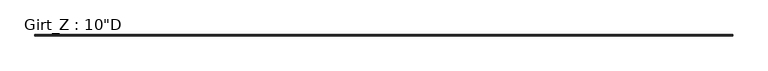
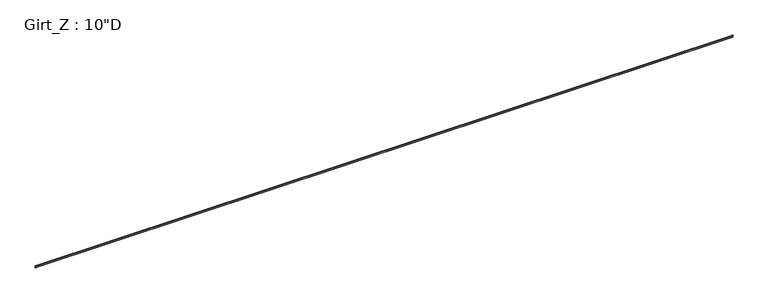
"""IFC4 building model written with IfcOpenShell, lengths in millimetres: beam geometry."""

from ifc_helpers import new_model, si_unit, point, frame, frame_2d, origin, place, context, project, spatial, polyline, circle_curve, trimmed, segment, composite_curve, outline, extrude, source, transform, mapped, element, save


def beam_b1d2936f(model_context):
    return source(origin(), model_context, "Body", "SweptSolid", [
        extrude(outline(composite_curve([segment(polyline([(-77.9859375, 127.0), (-3.3734375, 127.0)]), True, "CONTINUOUS"), segment(trimmed(circle_curve(frame_2d((-3.3734375, 122.2375)), 4.7625), [point((-3.3734375, 127.0))], [point((1.3890625, 122.2375))], False, "CARTESIAN"), True, "CONTINUOUS"), segment(polyline([(1.3890625, 122.2375), (1.3890625, -122.2389339)]), True, "CONTINUOUS"), segment(trimmed(circle_curve(frame_2d((3.3748024, -122.2389339)), 1.9857399), [point((1.3890625, -122.2389339))], [point((3.2694106, -124.221875))], True, "CARTESIAN"), True, "CONTINUOUS"), segment(polyline([(3.2694106, -124.221875), (83.0404765, -124.221875), (94.4528742, -110.621109), (96.5810415, -112.4068534), (84.3359375, -127.0), (-1.3890625, -127.0), (-1.3890625, 122.2381931)]), True, "CONTINUOUS"), segment(trimmed(circle_curve(frame_2d((-3.3741066, 122.2381931)), 1.9850441), [point((-1.3890625, 122.2381931))], [point((-3.3005807, 124.221875))], True, "CARTESIAN"), True, "CONTINUOUS"), segment(polyline([(-3.3005807, 124.221875), (-76.6904765, 124.221875), (-88.1028742, 110.621109), (-90.2310415, 112.4068534), (-77.9859375, 127.0)]), True, "CONTINUOUS")], self_intersect=False)), frame((-44221.4, 0.0, 0.0), z_axis=(1.0, 0.0, 0.0), x_axis=(0.0, 1.0, 0.0)), (0.0, 0.0, 1.0), 88442.8),
    ])


if __name__ == "__main__":
    model = new_model("IFC4")
    model_context = context("Model", 3, world=origin())
    ifc_project = project(units=[si_unit("LENGTHUNIT", "METRE", prefix="MILLI")], contexts=[model_context])
    site = spatial("IfcSite", under=ifc_project)
    building = spatial("IfcBuilding", under=site)
    placement = place(None, origin())
    beam_shape = beam_b1d2936f(model_context)
    element("IfcBeam", 1, ObjectType="Girt_Z : 10\"D", at=placement, inside=building, context=model_context, shape_type="MappedRepresentation", body=[
        mapped(beam_shape, transform((0.0, 0.0, 0.0), x_axis=(1.0, 0.0, 0.0), y_axis=(0.0, 1.0, 0.0), z_axis=(0.0, 0.0, 1.0))),
    ])
    save(model, "model.ifc")

# Revit data of these elements
# Type "Girt_Z : 10\"D"
#   half leg = 0' - 1 11/16"
#   Web_Thickness = 0' - 0 7/64"
#   Length [instance default] = 10' - 0"
#   Leg_2 = 0' - 3 3/8"
#   Leg_1 = 0' - 3 1/8"
#   Height = 0' - 10"
#   Structural Material [instance default] = none
# Element 1 (IfcBeam, "Girt_Z : 10\"D")
#   Structural Material = STRUCTURAL STEEL - SEE STRUCT. DWGS
#   Materials on its faces: "STRUCTURAL STEEL - SEE STRUCT. DWGS"
# Materials
#   "STRUCTURAL STEEL - SEE STRUCT. DWGS": class "Metal", colour RGB 137 146 153, transparency 0, Description = "Steel, mill finish", Cost = 0
